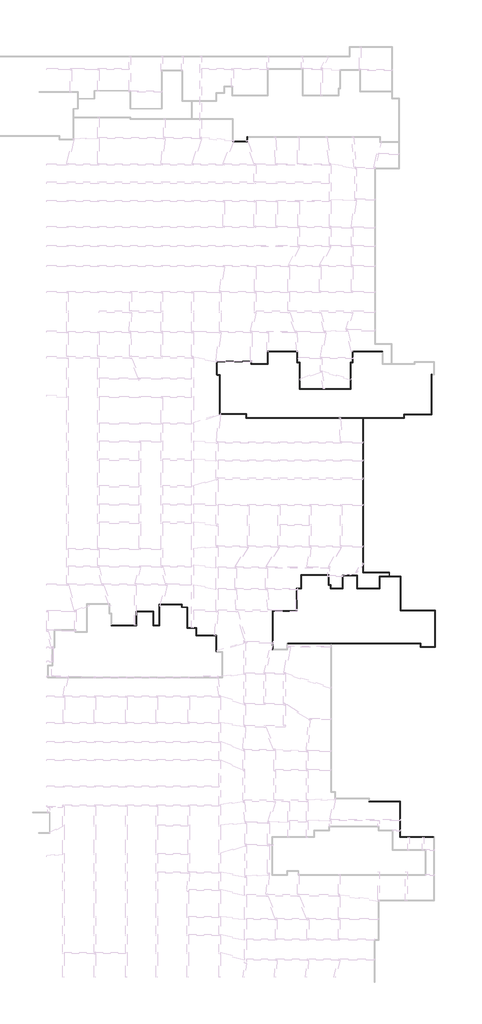
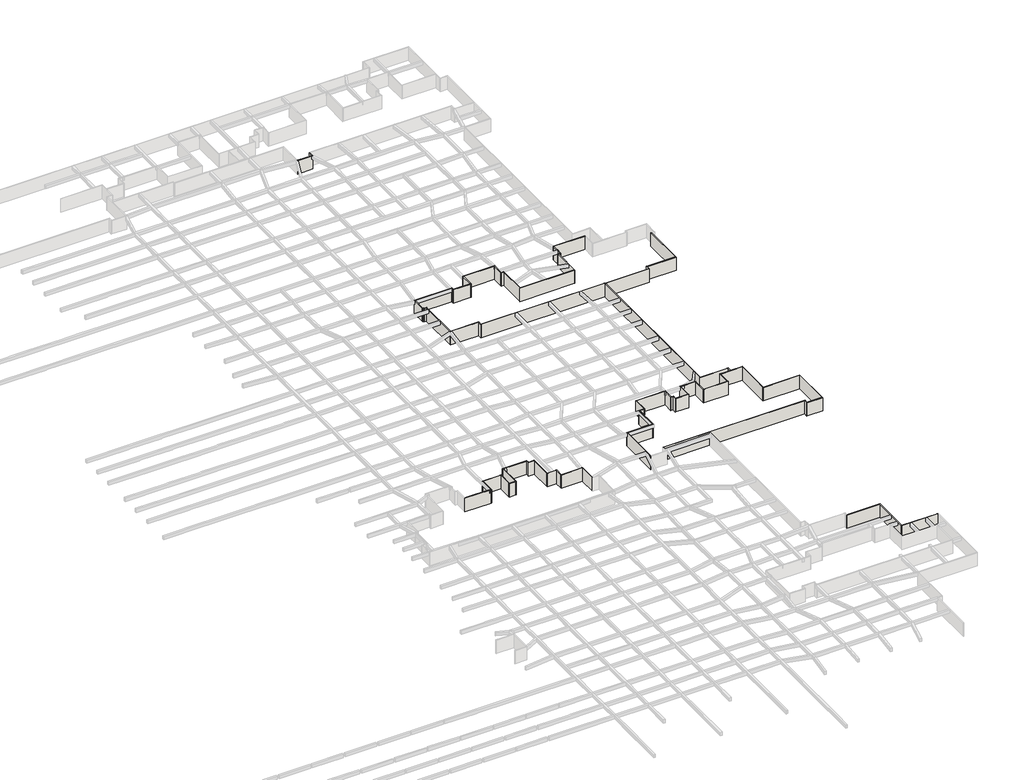
# One storey, part 9 of 45: 69 walls.
"""IFC4 building model written with IfcOpenShell, lengths in millimetres."""

from ifc_helpers import new_model, si_unit, origin, origin_with_axes, place, context, project, spatial, polyline, outline, extrude, faceted_brep, element, save

model = new_model("IFC4")

# Units and contexts
model_context = context("Model", 3, world=origin())
ifc_project = project(units=[si_unit("LENGTHUNIT", "METRE", prefix="MILLI")], contexts=[model_context])

# Site, building, storey
site = spatial("IfcSite", under=ifc_project)
building = spatial("IfcBuilding", under=site)
storey = spatial("IfcBuildingStorey", under=building, Name="户型图", Elevation=0.0)

# Walls
placement = place(None, origin())
element("IfcWall", 1, ObjectType="所有墙体", at=placement, inside=storey, context=model_context, shape_type="Brep", body=[
    faceted_brep([(78199.4783436, 16231.9876735, 0.0), (69819.4783436, 16231.9876735, 0.0), (69699.4783436, 16231.9876735, 0.0), (69699.4783436, 16231.9876735, 3300.0), (69819.4783436, 16231.9876735, 3300.0), (78199.4783436, 16231.9876735, 3300.0), (78199.4783436, 16111.9876735, 0.0), (78199.4783436, 16111.9876735, 3300.0), (69699.4783436, 16111.9876735, 3300.0), (69699.4783436, 16111.9876735, 0.0)], [[[0, 1, 2, 3, 4, 5]], [[6, 7, 8, 9]], [[2, 1, 0, 6, 9]], [[5, 4, 3, 8, 7]], [[0, 5, 7, 6]], [[3, 2, 9, 8]]]),
])
element("IfcWall", 2, ObjectType="所有墙体", at=placement, inside=storey, context=model_context, shape_type="Brep", body=[
    faceted_brep([(69819.4783436, 16231.9876735, 0.0), (69819.4783436, 25131.9876735, 0.0), (69819.4783436, 25131.9876735, 3300.0), (69819.4783436, 16231.9876735, 3300.0), (69699.4783436, 16231.9876735, 0.0), (69699.4783436, 16231.9876735, 3300.0), (69699.4783436, 25011.9876735, 3300.0), (69699.4783436, 25131.9876735, 3300.0), (69699.4783436, 25131.9876735, 0.0), (69699.4783436, 25011.9876735, 0.0)], [[[0, 1, 2, 3]], [[4, 5, 6, 7, 8, 9]], [[1, 0, 4, 9, 8]], [[3, 2, 7, 6, 5]], [[0, 3, 5, 4]], [[2, 1, 8, 7]]]),
])
element("IfcWall", 3, ObjectType="所有墙体", at=placement, inside=storey, context=model_context, shape_type="Brep", body=[
    faceted_brep([(69699.4783436, 25131.9876735, 0.0), (62019.4783436, 25131.9876735, 0.0), (61899.4783436, 25131.9876735, 0.0), (61899.4783436, 25131.9876735, 3300.0), (62019.4783436, 25131.9876735, 3300.0), (69699.4783436, 25131.9876735, 3300.0), (69699.4783436, 25011.9876735, 0.0), (69699.4783436, 25011.9876735, 3300.0), (61899.4783436, 25011.9876735, 3300.0), (61899.4783436, 25011.9876735, 0.0)], [[[0, 1, 2, 3, 4, 5]], [[6, 7, 8, 9]], [[2, 1, 0, 6, 9]], [[5, 4, 3, 8, 7]], [[0, 5, 7, 6]], [[3, 2, 9, 8]]]),
])
element("IfcWall", 4, ObjectType="所有墙体", at=placement, inside=storey, context=model_context, shape_type="Brep", body=[
    faceted_brep([(41607.3862954, 64511.9876735, 0.0), (52399.4783436, 64511.9876735, 0.0), (52519.4783436, 64511.9876735, 0.0), (74799.4783436, 64511.9876735, 0.0), (74919.4783436, 64511.9876735, 0.0), (74919.4783436, 64511.9876735, 3300.0), (74799.4783436, 64511.9876735, 3300.0), (52519.4783436, 64511.9876735, 3300.0), (52399.4783436, 64511.9876735, 3300.0), (41607.3862954, 64511.9876735, 3300.0), (41607.3862954, 64631.9876735, 0.0), (41607.3862954, 64631.9876735, 3300.0), (74919.4783436, 64631.9876735, 3300.0), (74919.4783436, 64631.9876735, 0.0)], [[[0, 1, 2, 3, 4, 5, 6, 7, 8, 9]], [[10, 11, 12, 13]], [[4, 3, 2, 1, 0, 10, 13]], [[9, 8, 7, 6, 5, 12, 11]], [[5, 4, 13, 12]], [[0, 9, 11, 10]]]),
])
element("IfcWall", 5, ObjectType="所有墙体", at=placement, inside=storey, context=model_context, shape_type="Brep", body=[
    faceted_brep([(74799.4783436, 64511.9876735, 0.0), (74799.4783436, 63611.9876735, 0.0), (74799.4783436, 63611.9876735, 3300.0), (74799.4783436, 64511.9876735, 3300.0), (74919.4783436, 64511.9876735, 0.0), (74919.4783436, 64511.9876735, 3300.0), (74919.4783436, 63731.9876735, 3300.0), (74919.4783436, 63611.9876735, 3300.0), (74919.4783436, 63611.9876735, 0.0), (74919.4783436, 63731.9876735, 0.0)], [[[0, 1, 2, 3]], [[4, 5, 6, 7, 8, 9]], [[1, 0, 4, 9, 8]], [[3, 2, 7, 6, 5]], [[0, 3, 5, 4]], [[2, 1, 8, 7]]]),
])
element("IfcWall", 6, ObjectType="所有墙体", at=placement, inside=storey, context=model_context, shape_type="Brep", body=[
    faceted_brep([(74919.4783436, 63611.9876735, 0.0), (78519.4783436, 63611.9876735, 0.0), (78519.4783436, 63611.9876735, 3300.0), (74919.4783436, 63611.9876735, 3300.0), (74919.4783436, 63731.9876735, 0.0), (74919.4783436, 63731.9876735, 3300.0), (78399.4783436, 63731.9876735, 3300.0), (78519.4783436, 63731.9876735, 3300.0), (78519.4783436, 63731.9876735, 0.0), (78399.4783436, 63731.9876735, 0.0)], [[[0, 1, 2, 3]], [[4, 5, 6, 7, 8, 9]], [[1, 0, 4, 9, 8]], [[3, 2, 7, 6, 5]], [[0, 3, 5, 4]], [[2, 1, 8, 7]]]),
])
element("IfcWall", 7, ObjectType="所有墙体", at=placement, inside=storey, context=model_context, shape_type="Brep", body=[
    faceted_brep([(78519.4783436, 63731.9876735, 0.0), (78519.4783436, 72831.9876735, 0.0), (78519.4783436, 72831.9876735, 3300.0), (78519.4783436, 63731.9876735, 3300.0), (78399.4783436, 63731.9876735, 0.0), (78399.4783436, 63731.9876735, 3300.0), (78399.4783436, 72711.9876735, 3300.0), (78399.4783436, 72831.9876735, 3300.0), (78399.4783436, 72831.9876735, 0.0), (78399.4783436, 72711.9876735, 0.0)], [[[0, 1, 2, 3]], [[4, 5, 6, 7, 8, 9]], [[1, 0, 4, 9, 8]], [[3, 2, 7, 6, 5]], [[0, 3, 5, 4]], [[2, 1, 8, 7]]]),
])
element("IfcWall", 8, ObjectType="所有墙体", at=placement, inside=storey, context=model_context, shape_type="Brep", body=[
    faceted_brep([(78399.4783436, 72831.9876735, 0.0), (69919.4783436, 72831.9876735, 0.0), (69799.4783436, 72831.9876735, 0.0), (69799.4783436, 72831.9876735, 3300.0), (69919.4783436, 72831.9876735, 3300.0), (78399.4783436, 72831.9876735, 3300.0), (78399.4783436, 72711.9876735, 0.0), (78399.4783436, 72711.9876735, 3300.0), (69799.4783436, 72711.9876735, 3300.0), (69799.4783436, 72711.9876735, 0.0)], [[[0, 1, 2, 3, 4, 5]], [[6, 7, 8, 9]], [[2, 1, 0, 6, 9]], [[5, 4, 3, 8, 7]], [[0, 5, 7, 6]], [[3, 2, 9, 8]]]),
])
element("IfcWall", 9, ObjectType="所有墙体", at=placement, inside=storey, context=model_context, shape_type="Brep", body=[
    faceted_brep([(69919.4783436, 72831.9876735, 0.0), (69919.4783436, 81331.9876735, 0.0), (69919.4783436, 81331.9876735, 3300.0), (69919.4783436, 72831.9876735, 3300.0), (69799.4783436, 72831.9876735, 0.0), (69799.4783436, 72831.9876735, 3300.0), (69799.4783436, 81211.9876735, 3300.0), (69799.4783436, 81331.9876735, 3300.0), (69799.4783436, 81331.9876735, 0.0), (69799.4783436, 81211.9876735, 0.0)], [[[0, 1, 2, 3]], [[4, 5, 6, 7, 8, 9]], [[1, 0, 4, 9, 8]], [[3, 2, 7, 6, 5]], [[0, 3, 5, 4]], [[2, 1, 8, 7]]]),
])
element("IfcWall", 10, ObjectType="所有墙体", at=placement, inside=storey, context=model_context, shape_type="Brep", body=[
    faceted_brep([(69799.4783436, 81331.9876735, 0.0), (67119.4783436, 81331.9876735, 0.0), (66999.4783436, 81331.9876735, 0.0), (64738.2147368, 81331.9876735, 0.0), (64738.2147368, 81331.9876735, 3300.0), (66999.4783436, 81331.9876735, 3300.0), (67119.4783436, 81331.9876735, 3300.0), (69799.4783436, 81331.9876735, 3300.0), (69799.4783436, 81211.9876735, 0.0), (69799.4783436, 81211.9876735, 3300.0), (64738.2147368, 81211.9876735, 3300.0), (64738.2147368, 81211.9876735, 0.0)], [[[0, 1, 2, 3, 4, 5, 6, 7]], [[8, 9, 10, 11]], [[3, 2, 1, 0, 8, 11]], [[7, 6, 5, 4, 10, 9]], [[0, 7, 9, 8]], [[4, 3, 11, 10]]]),
])
element("IfcWall", 11, ObjectType="所有墙体", at=placement, inside=storey, context=model_context, shape_type="Brep", body=[
    faceted_brep([(67119.4783436, 81331.9876735, 0.0), (67119.4783436, 82331.9876735, 0.0), (67119.4783436, 82331.9876735, 3300.0), (67119.4783436, 81331.9876735, 3300.0), (66999.4783436, 81331.9876735, 0.0), (66999.4783436, 81331.9876735, 3300.0), (66999.4783436, 82211.9876735, 3300.0), (66999.4783436, 82331.9876735, 3300.0), (66999.4783436, 82331.9876735, 0.0), (66999.4783436, 82211.9876735, 0.0)], [[[0, 1, 2, 3]], [[4, 5, 6, 7, 8, 9]], [[1, 0, 4, 9, 8]], [[3, 2, 7, 6, 5]], [[0, 3, 5, 4]], [[2, 1, 8, 7]]]),
])
element("IfcWall", 12, ObjectType="所有墙体", at=placement, inside=storey, context=model_context, shape_type="Brep", body=[
    faceted_brep([(66999.4783436, 82331.9876735, 0.0), (60519.4783436, 82331.9876735, 0.0), (60399.4783436, 82331.9876735, 0.0), (60399.4783436, 82331.9876735, 3300.0), (60519.4783436, 82331.9876735, 3300.0), (66999.4783436, 82331.9876735, 3300.0), (66999.4783436, 82211.9876735, 0.0), (66999.4783436, 82211.9876735, 3300.0), (60399.4783436, 82211.9876735, 3300.0), (60399.4783436, 82211.9876735, 0.0)], [[[0, 1, 2, 3, 4, 5]], [[6, 7, 8, 9]], [[2, 1, 0, 6, 9]], [[5, 4, 3, 8, 7]], [[0, 5, 7, 6]], [[3, 2, 9, 8]]]),
])
element("IfcWall", 13, ObjectType="所有墙体", at=placement, inside=storey, context=model_context, shape_type="Brep", body=[
    faceted_brep([(60519.4783436, 82331.9876735, 0.0), (60519.4783436, 120811.9876735, 0.0), (60519.4783436, 120931.9876735, 0.0), (60519.4783436, 120931.9876735, 3300.0), (60519.4783436, 120811.9876735, 3300.0), (60519.4783436, 82331.9876735, 3300.0), (60399.4783436, 82331.9876735, 0.0), (60399.4783436, 82331.9876735, 3300.0), (60399.4783436, 120846.7035402, 3300.0), (60399.4783436, 120931.9876735, 3300.0), (60399.4783436, 120931.9876735, 0.0), (60399.4783436, 120846.7035402, 0.0)], [[[0, 1, 2, 3, 4, 5]], [[6, 7, 8, 9, 10, 11]], [[2, 1, 0, 6, 11, 10]], [[5, 4, 3, 9, 8, 7]], [[0, 5, 7, 6]], [[3, 2, 10, 9]]]),
])
element("IfcWall", 14, ObjectType="所有墙体", at=placement, inside=storey, context=model_context, shape_type="Brep", body=[
    faceted_brep([(60519.4783436, 120811.9876735, 0.0), (70819.4783436, 120811.9876735, 0.0), (70819.4783436, 120811.9876735, 3300.0), (60519.4783436, 120811.9876735, 3300.0), (60519.4783436, 120931.9876735, 0.0), (60519.4783436, 120931.9876735, 3300.0), (70699.4783436, 120931.9876735, 3300.0), (70819.4783436, 120931.9876735, 3300.0), (70819.4783436, 120931.9876735, 0.0), (70699.4783436, 120931.9876735, 0.0)], [[[0, 1, 2, 3]], [[4, 5, 6, 7, 8, 9]], [[1, 0, 4, 9, 8]], [[3, 2, 7, 6, 5]], [[0, 3, 5, 4]], [[2, 1, 8, 7]]]),
])
element("IfcWall", 15, ObjectType="所有墙体", at=placement, inside=storey, context=model_context, shape_type="Brep", body=[
    faceted_brep([(70819.4783436, 120931.9876735, 0.0), (70819.4783436, 121711.9876735, 0.0), (70819.4783436, 121831.9876735, 0.0), (70819.4783436, 121831.9876735, 3300.0), (70819.4783436, 121711.9876735, 3300.0), (70819.4783436, 120931.9876735, 3300.0), (70699.4783436, 120931.9876735, 0.0), (70699.4783436, 120931.9876735, 3300.0), (70699.4783436, 121831.9876735, 3300.0), (70699.4783436, 121831.9876735, 0.0)], [[[0, 1, 2, 3, 4, 5]], [[6, 7, 8, 9]], [[2, 1, 0, 6, 9]], [[5, 4, 3, 8, 7]], [[0, 5, 7, 6]], [[3, 2, 9, 8]]]),
])
element("IfcWall", 16, ObjectType="所有墙体", at=placement, inside=storey, context=model_context, shape_type="Brep", body=[
    faceted_brep([(70819.4783436, 121711.9876735, 0.0), (77619.4783436, 121711.9876735, 0.0), (77619.4783436, 121711.9876735, 3300.0), (70819.4783436, 121711.9876735, 3300.0), (70819.4783436, 121831.9876735, 0.0), (70819.4783436, 121831.9876735, 3300.0), (77499.4783436, 121831.9876735, 3300.0), (77619.4783436, 121831.9876735, 3300.0), (77619.4783436, 121831.9876735, 0.0), (77499.4783436, 121831.9876735, 0.0)], [[[0, 1, 2, 3]], [[4, 5, 6, 7, 8, 9]], [[1, 0, 4, 9, 8]], [[3, 2, 7, 6, 5]], [[0, 3, 5, 4]], [[2, 1, 8, 7]]]),
])
element("IfcWall", 17, ObjectType="所有墙体", at=placement, inside=storey, context=model_context, shape_type="Brep", body=[
    faceted_brep([(77619.4783436, 121831.9876735, 0.0), (77619.4783436, 131611.9876735, 0.0), (77619.4783436, 131731.9876735, 0.0), (77619.4783436, 131731.9876735, 3300.0), (77619.4783436, 131611.9876735, 3300.0), (77619.4783436, 121831.9876735, 3300.0), (77499.4783436, 121831.9876735, 0.0), (77499.4783436, 121831.9876735, 3300.0), (77499.4783436, 131731.9876735, 3300.0), (77499.4783436, 131731.9876735, 0.0)], [[[0, 1, 2, 3, 4, 5]], [[6, 7, 8, 9]], [[2, 1, 0, 6, 9]], [[5, 4, 3, 8, 7]], [[0, 5, 7, 6]], [[3, 2, 9, 8]]]),
])
element("IfcWall", 18, ObjectType="所有墙体", at=placement, inside=storey, context=model_context, shape_type="Brep", body=[
    faceted_brep([(27971.0399311, 189831.009409, 0.0), (31556.641355, 189831.009409, 0.0), (31556.641355, 189831.009409, 3300.0), (27971.0399311, 189831.009409, 3300.0), (27971.0399311, 189951.009409, 0.0), (27971.0399311, 189951.009409, 3300.0), (31436.641355, 189951.009409, 3300.0), (31556.641355, 189951.009409, 3300.0), (31556.641355, 189951.009409, 0.0), (31436.641355, 189951.009409, 0.0)], [[[0, 1, 2, 3]], [[4, 5, 6, 7, 8, 9]], [[1, 0, 4, 9, 8]], [[3, 2, 7, 6, 5]], [[0, 3, 5, 4]], [[2, 1, 8, 7]]]),
])
element("IfcWall", 19, ObjectType="所有墙体", at=placement, inside=storey, context=model_context, shape_type="Brep", body=[
    faceted_brep([(31556.641355, 189951.009409, 0.0), (31556.641355, 191031.009409, 0.0), (31556.641355, 191151.009409, 0.0), (31556.641355, 191151.009409, 3300.0), (31556.641355, 191031.009409, 3300.0), (31556.641355, 189951.009409, 3300.0), (31436.641355, 189951.009409, 0.0), (31436.641355, 189951.009409, 3300.0), (31436.641355, 191151.009409, 3300.0), (31436.641355, 191151.009409, 0.0)], [[[0, 1, 2, 3, 4, 5]], [[6, 7, 8, 9]], [[2, 1, 0, 6, 9]], [[5, 4, 3, 8, 7]], [[0, 5, 7, 6]], [[3, 2, 9, 8]]]),
])
element("IfcWall", 20, ObjectType="所有墙体", at=placement, inside=storey, context=model_context, shape_type="Brep", body=[
    faceted_brep([(23805.9205959, 135031.9876735, 0.0), (23805.9205959, 131823.6321803, 0.0), (23805.9205959, 131823.6321803, 3300.0), (23805.9205959, 135031.9876735, 3300.0), (23925.9205959, 135031.9876735, 0.0), (23925.9205959, 135031.9876735, 3300.0), (23925.9205959, 134911.9876735, 3300.0), (23925.9205959, 131823.6321803, 3300.0), (23925.9205959, 131823.6321803, 0.0), (23925.9205959, 134911.9876735, 0.0)], [[[0, 1, 2, 3]], [[4, 5, 6, 7, 8, 9]], [[1, 0, 4, 9, 8]], [[3, 2, 7, 6, 5]], [[2, 1, 8, 7]], [[0, 3, 5, 4]]]),
])
element("IfcWall", 21, ObjectType="所有墙体", at=placement, inside=storey, context=model_context, shape_type="Brep", body=[
    faceted_brep([(23805.9205959, 131703.6321803, 0.0), (24005.9205959, 131703.6321803, 0.0), (24125.9205959, 131703.6321803, 0.0), (24125.9205959, 131703.6321803, 3300.0), (24005.9205959, 131703.6321803, 3300.0), (23805.9205959, 131703.6321803, 3300.0), (23805.9205959, 131823.6321803, 0.0), (23805.9205959, 131823.6321803, 3300.0), (23925.9205959, 131823.6321803, 3300.0), (24125.9205959, 131823.6321803, 3300.0), (24125.9205959, 131823.6321803, 0.0), (23925.9205959, 131823.6321803, 0.0)], [[[0, 1, 2, 3, 4, 5]], [[6, 7, 8, 9, 10, 11]], [[2, 1, 0, 6, 11, 10]], [[5, 4, 3, 9, 8, 7]], [[0, 5, 7, 6]], [[3, 2, 10, 9]]]),
])
element("IfcWall", 22, ObjectType="所有墙体", at=placement, inside=storey, context=model_context, shape_type="Brep", body=[
    faceted_brep([(24005.9205959, 131703.6321803, 0.0), (24005.9205959, 131503.6321803, 0.0), (24005.9205959, 131503.6321803, 3300.0), (24005.9205959, 131703.6321803, 3300.0), (24125.9205959, 131703.6321803, 0.0), (24125.9205959, 131703.6321803, 3300.0), (24125.9205959, 131623.6321803, 3300.0), (24125.9205959, 131503.6321803, 3300.0), (24125.9205959, 131503.6321803, 0.0), (24125.9205959, 131623.6321803, 0.0)], [[[0, 1, 2, 3]], [[4, 5, 6, 7, 8, 9]], [[1, 0, 4, 9, 8]], [[3, 2, 7, 6, 5]], [[0, 3, 5, 4]], [[2, 1, 8, 7]]]),
])
element("IfcWall", 23, ObjectType="所有墙体", at=placement, inside=storey, context=model_context, shape_type="Brep", body=[
    faceted_brep([(24125.9205959, 131503.6321803, 0.0), (24605.9205959, 131503.6321803, 0.0), (24725.9205959, 131503.6321803, 0.0), (24725.9205959, 131503.6321803, 3300.0), (24605.9205959, 131503.6321803, 3300.0), (24125.9205959, 131503.6321803, 3300.0), (24125.9205959, 131623.6321803, 0.0), (24125.9205959, 131623.6321803, 3300.0), (24725.9205959, 131623.6321803, 3300.0), (24725.9205959, 131623.6321803, 0.0)], [[[0, 1, 2, 3, 4, 5]], [[6, 7, 8, 9]], [[2, 1, 0, 6, 9]], [[5, 4, 3, 8, 7]], [[0, 5, 7, 6]], [[3, 2, 9, 8]]]),
])
element("IfcWall", 24, ObjectType="所有墙体", at=placement, inside=storey, context=model_context, shape_type="Brep", body=[
    faceted_brep([(24605.9205959, 131503.6321803, 0.0), (24605.9205959, 121746.7035402, 0.0), (24605.9205959, 121746.7035402, 3300.0), (24605.9205959, 131503.6321803, 3300.0), (24725.9205959, 131503.6321803, 0.0), (24725.9205959, 131503.6321803, 3300.0), (24725.9205959, 121866.7035402, 3300.0), (24725.9205959, 121746.7035402, 3300.0), (24725.9205959, 121746.7035402, 0.0), (24725.9205959, 121866.7035402, 0.0)], [[[0, 1, 2, 3]], [[4, 5, 6, 7, 8, 9]], [[1, 0, 4, 9, 8]], [[3, 2, 7, 6, 5]], [[0, 3, 5, 4]], [[2, 1, 8, 7]]]),
])
element("IfcWall", 25, ObjectType="所有墙体", at=placement, inside=storey, context=model_context, shape_type="Brep", body=[
    faceted_brep([(24725.9205959, 121746.7035402, 0.0), (31205.9205959, 121746.7035402, 0.0), (31325.9205959, 121746.7035402, 0.0), (31325.9205959, 121746.7035402, 3300.0), (31205.9205959, 121746.7035402, 3300.0), (24725.9205959, 121746.7035402, 3300.0), (24725.9205959, 121866.7035402, 0.0), (24725.9205959, 121866.7035402, 3300.0), (31325.9205959, 121866.7035402, 3300.0), (31325.9205959, 121866.7035402, 0.0)], [[[0, 1, 2, 3, 4, 5]], [[6, 7, 8, 9]], [[2, 1, 0, 6, 9]], [[5, 4, 3, 8, 7]], [[0, 5, 7, 6]], [[3, 2, 9, 8]]]),
])
element("IfcWall", 26, ObjectType="所有墙体", at=placement, inside=storey, context=model_context, shape_type="Brep", body=[
    faceted_brep([(31205.9205959, 121746.7035402, 0.0), (31205.9205959, 120846.7035402, 0.0), (31205.9205959, 120846.7035402, 3300.0), (31205.9205959, 121746.7035402, 3300.0), (31325.9205959, 121746.7035402, 0.0), (31325.9205959, 121746.7035402, 3300.0), (31325.9205959, 120966.7035402, 3300.0), (31325.9205959, 120846.7035402, 3300.0), (31325.9205959, 120846.7035402, 0.0), (31325.9205959, 120966.7035402, 0.0)], [[[0, 1, 2, 3]], [[4, 5, 6, 7, 8, 9]], [[1, 0, 4, 9, 8]], [[3, 2, 7, 6, 5]], [[0, 3, 5, 4]], [[2, 1, 8, 7]]]),
])
element("IfcWall", 27, ObjectType="所有墙体", at=placement, inside=storey, context=model_context, shape_type="Brep", body=[
    faceted_brep([(31325.9205959, 120846.7035402, 0.0), (60399.4783436, 120846.7035402, 0.0), (60399.4783436, 120846.7035402, 3300.0), (31325.9205959, 120846.7035402, 3300.0), (31325.9205959, 120966.7035402, 0.0), (31325.9205959, 120966.7035402, 3300.0), (60399.4783436, 120966.7035402, 3300.0), (60399.4783436, 120966.7035402, 0.0), (60399.4783436, 120931.9876735, 0.0), (60399.4783436, 120931.9876735, 3300.0)], [[[0, 1, 2, 3]], [[4, 5, 6, 7]], [[1, 0, 4, 7, 8]], [[3, 2, 9, 6, 5]], [[0, 3, 5, 4]], [[2, 1, 8, 7, 6, 9]]]),
])
element("IfcWall", 28, ObjectType="所有墙体", at=placement, inside=storey, context=model_context, shape_type="Brep", body=[
    faceted_brep([(65299.4783436, 137531.9876735, 0.0), (57865.3118233, 137531.9876735, 0.0), (57865.3118233, 137531.9876735, 3300.0), (65299.4783436, 137531.9876735, 3300.0), (65299.4783436, 137411.9876735, 0.0), (65299.4783436, 137411.9876735, 3300.0), (57985.3118233, 137411.9876735, 3300.0), (57865.3118233, 137411.9876735, 3300.0), (57865.3118233, 137411.9876735, 0.0), (57985.3118233, 137411.9876735, 0.0)], [[[0, 1, 2, 3]], [[4, 5, 6, 7, 8, 9]], [[1, 0, 4, 9, 8]], [[3, 2, 7, 6, 5]], [[0, 3, 5, 4]], [[2, 1, 8, 7]]]),
])
element("IfcWall", 29, ObjectType="所有墙体", at=placement, inside=storey, context=model_context, shape_type="Brep", body=[
    faceted_brep([(57865.3118233, 137411.9876735, 0.0), (57865.3118233, 134731.9876735, 0.0), (57865.3118233, 134611.9876735, 0.0), (57865.3118233, 134611.9876735, 3300.0), (57865.3118233, 134731.9876735, 3300.0), (57865.3118233, 137411.9876735, 3300.0), (57985.3118233, 137411.9876735, 0.0), (57985.3118233, 137411.9876735, 3300.0), (57985.3118233, 134611.9876735, 3300.0), (57985.3118233, 134611.9876735, 0.0)], [[[0, 1, 2, 3, 4, 5]], [[6, 7, 8, 9]], [[2, 1, 0, 6, 9]], [[5, 4, 3, 8, 7]], [[0, 5, 7, 6]], [[3, 2, 9, 8]]]),
])
element("IfcWall", 30, ObjectType="所有墙体", at=placement, inside=storey, context=model_context, shape_type="Brep", body=[
    faceted_brep([(57865.3118233, 134731.9876735, 0.0), (57365.3118233, 134731.9876735, 0.0), (57365.3118233, 134731.9876735, 3300.0), (57865.3118233, 134731.9876735, 3300.0), (57865.3118233, 134611.9876735, 0.0), (57865.3118233, 134611.9876735, 3300.0), (57485.3118233, 134611.9876735, 3300.0), (57365.3118233, 134611.9876735, 3300.0), (57365.3118233, 134611.9876735, 0.0), (57485.3118233, 134611.9876735, 0.0)], [[[0, 1, 2, 3]], [[4, 5, 6, 7, 8, 9]], [[1, 0, 4, 9, 8]], [[3, 2, 7, 6, 5]], [[0, 3, 5, 4]], [[2, 1, 8, 7]]]),
])
element("IfcWall", 31, ObjectType="所有墙体", at=placement, inside=storey, context=model_context, shape_type="Brep", body=[
    faceted_brep([(57365.3118233, 134611.9876735, 0.0), (57365.3118233, 128131.9876735, 0.0), (57365.3118233, 128011.9876735, 0.0), (57365.3118233, 128011.9876735, 3300.0), (57365.3118233, 128131.9876735, 3300.0), (57365.3118233, 134611.9876735, 3300.0), (57485.3118233, 134611.9876735, 0.0), (57485.3118233, 134611.9876735, 3300.0), (57485.3118233, 128011.9876735, 3300.0), (57485.3118233, 128011.9876735, 0.0)], [[[0, 1, 2, 3, 4, 5]], [[6, 7, 8, 9]], [[2, 1, 0, 6, 9]], [[5, 4, 3, 8, 7]], [[0, 5, 7, 6]], [[3, 2, 9, 8]]]),
])
element("IfcWall", 32, ObjectType="所有墙体", at=placement, inside=storey, context=model_context, shape_type="Brep", body=[
    faceted_brep([(57365.3118233, 128131.9876735, 0.0), (44685.3118233, 128131.9876735, 0.0), (44565.3118233, 128131.9876735, 0.0), (44565.3118233, 128131.9876735, 3300.0), (44685.3118233, 128131.9876735, 3300.0), (57365.3118233, 128131.9876735, 3300.0), (57365.3118233, 128011.9876735, 0.0), (57365.3118233, 128011.9876735, 3300.0), (44565.3118233, 128011.9876735, 3300.0), (44565.3118233, 128011.9876735, 0.0)], [[[0, 1, 2, 3, 4, 5]], [[6, 7, 8, 9]], [[2, 1, 0, 6, 9]], [[5, 4, 3, 8, 7]], [[0, 5, 7, 6]], [[3, 2, 9, 8]]]),
])
element("IfcWall", 33, ObjectType="所有墙体", at=placement, inside=storey, context=model_context, shape_type="Brep", body=[
    faceted_brep([(44685.3118233, 128131.9876735, 0.0), (44685.3118233, 134731.9876735, 0.0), (44685.3118233, 134731.9876735, 3300.0), (44685.3118233, 128131.9876735, 3300.0), (44565.3118233, 128131.9876735, 0.0), (44565.3118233, 128131.9876735, 3300.0), (44565.3118233, 134611.9876735, 3300.0), (44565.3118233, 134731.9876735, 3300.0), (44565.3118233, 134731.9876735, 0.0), (44565.3118233, 134611.9876735, 0.0)], [[[0, 1, 2, 3]], [[4, 5, 6, 7, 8, 9]], [[1, 0, 4, 9, 8]], [[3, 2, 7, 6, 5]], [[0, 3, 5, 4]], [[2, 1, 8, 7]]]),
])
element("IfcWall", 34, ObjectType="所有墙体", at=placement, inside=storey, context=model_context, shape_type="Brep", body=[
    faceted_brep([(44565.3118233, 134731.9876735, 0.0), (44085.3118233, 134731.9876735, 0.0), (43965.3118233, 134731.9876735, 0.0), (43965.3118233, 134731.9876735, 3300.0), (44085.3118233, 134731.9876735, 3300.0), (44565.3118233, 134731.9876735, 3300.0), (44565.3118233, 134611.9876735, 0.0), (44565.3118233, 134611.9876735, 3300.0), (43965.3118233, 134611.9876735, 3300.0), (43965.3118233, 134611.9876735, 0.0)], [[[0, 1, 2, 3, 4, 5]], [[6, 7, 8, 9]], [[2, 1, 0, 6, 9]], [[5, 4, 3, 8, 7]], [[0, 5, 7, 6]], [[3, 2, 9, 8]]]),
])
element("IfcWall", 35, ObjectType="所有墙体", at=placement, inside=storey, context=model_context, shape_type="Brep", body=[
    faceted_brep([(44085.3118233, 134731.9876735, 0.0), (44085.3118233, 137531.9876735, 0.0), (44085.3118233, 137531.9876735, 3300.0), (44085.3118233, 134731.9876735, 3300.0), (43965.3118233, 134731.9876735, 0.0), (43965.3118233, 134731.9876735, 3300.0), (43965.3118233, 137411.9876735, 3300.0), (43965.3118233, 137531.9876735, 3300.0), (43965.3118233, 137531.9876735, 0.0), (43965.3118233, 137411.9876735, 0.0)], [[[0, 1, 2, 3]], [[4, 5, 6, 7, 8, 9]], [[1, 0, 4, 9, 8]], [[3, 2, 7, 6, 5]], [[0, 3, 5, 4]], [[2, 1, 8, 7]]]),
])
element("IfcWall", 36, ObjectType="所有墙体", at=placement, inside=storey, context=model_context, shape_type="Brep", body=[
    faceted_brep([(43965.3118233, 137531.9876735, 0.0), (36602.5542012, 137531.9876735, 0.0), (36602.5542012, 137531.9876735, 3300.0), (43965.3118233, 137531.9876735, 3300.0), (43965.3118233, 137411.9876735, 0.0), (43965.3118233, 137411.9876735, 3300.0), (36722.5542012, 137411.9876735, 3300.0), (36602.5542012, 137411.9876735, 3300.0), (36602.5542012, 137411.9876735, 0.0), (36722.5542012, 137411.9876735, 0.0)], [[[0, 1, 2, 3]], [[4, 5, 6, 7, 8, 9]], [[1, 0, 4, 9, 8]], [[3, 2, 7, 6, 5]], [[0, 3, 5, 4]], [[2, 1, 8, 7]]]),
])
element("IfcWall", 37, ObjectType="所有墙体", at=placement, inside=storey, context=model_context, shape_type="Brep", body=[
    faceted_brep([(36602.5542012, 137411.9876735, 0.0), (36602.5542012, 134431.9876735, 0.0), (36602.5542012, 134311.9876735, 0.0), (36602.5542012, 134311.9876735, 3300.0), (36602.5542012, 134431.9876735, 3300.0), (36602.5542012, 137411.9876735, 3300.0), (36722.5542012, 137411.9876735, 0.0), (36722.5542012, 137411.9876735, 3300.0), (36722.5542012, 134311.9876735, 3300.0), (36722.5542012, 134311.9876735, 0.0)], [[[0, 1, 2, 3, 4, 5]], [[6, 7, 8, 9]], [[2, 1, 0, 6, 9]], [[5, 4, 3, 8, 7]], [[0, 5, 7, 6]], [[3, 2, 9, 8]]]),
])
element("IfcWall", 38, ObjectType="所有墙体", at=placement, inside=storey, context=model_context, shape_type="Brep", body=[
    faceted_brep([(36602.5542012, 134431.9876735, 0.0), (32622.5542012, 134431.9876735, 0.0), (32502.5542012, 134431.9876735, 0.0), (32502.5542012, 134431.9876735, 3300.0), (32622.5542012, 134431.9876735, 3300.0), (36602.5542012, 134431.9876735, 3300.0), (36602.5542012, 134311.9876735, 0.0), (36602.5542012, 134311.9876735, 3300.0), (32502.5542012, 134311.9876735, 3300.0), (32502.5542012, 134311.9876735, 0.0)], [[[0, 1, 2, 3, 4, 5]], [[6, 7, 8, 9]], [[2, 1, 0, 6, 9]], [[5, 4, 3, 8, 7]], [[0, 5, 7, 6]], [[3, 2, 9, 8]]]),
])
element("IfcWall", 39, ObjectType="所有墙体", at=placement, inside=storey, context=model_context, shape_type="Brep", body=[
    faceted_brep([(32622.5542012, 134431.9876735, 0.0), (32622.5542012, 135031.9876735, 0.0), (32622.5542012, 135031.9876735, 3300.0), (32622.5542012, 134431.9876735, 3300.0), (32502.5542012, 134431.9876735, 0.0), (32502.5542012, 134431.9876735, 3300.0), (32502.5542012, 134911.9876735, 3300.0), (32502.5542012, 135031.9876735, 3300.0), (32502.5542012, 135031.9876735, 0.0), (32502.5542012, 134911.9876735, 0.0)], [[[0, 1, 2, 3]], [[4, 5, 6, 7, 8, 9]], [[1, 0, 4, 9, 8]], [[3, 2, 7, 6, 5]], [[0, 3, 5, 4]], [[2, 1, 8, 7]]]),
])
element("IfcWall", 40, ObjectType="所有墙体", at=placement, inside=storey, context=model_context, shape_type="SweptSolid", body=[
    extrude(outline(polyline([(23925.9205959, 135031.9876735), (32502.5542012, 135031.9876735), (32502.5542012, 134911.9876735), (23925.9205959, 134911.9876735), (23925.9205959, 135031.9876735)])), origin_with_axes(), (0.0, 0.0, 1.0), 3300.0),
])
element("IfcWall", 41, ObjectType="所有墙体", at=placement, inside=storey, context=model_context, shape_type="Brep", body=[
    faceted_brep([(44987.3862954, 81638.4446559, 0.0), (44987.3862954, 78338.4446559, 0.0), (44987.3862954, 78218.4446559, 0.0), (44987.3862954, 78218.4446559, 3300.0), (44987.3862954, 78338.4446559, 3300.0), (44987.3862954, 81638.4446559, 3300.0), (45107.3862954, 81638.4446559, 0.0), (45107.3862954, 81638.4446559, 3300.0), (45107.3862954, 81518.4446559, 3300.0), (45107.3862954, 78218.4446559, 3300.0), (45107.3862954, 78218.4446559, 0.0), (45107.3862954, 81518.4446559, 0.0)], [[[0, 1, 2, 3, 4, 5]], [[6, 7, 8, 9, 10, 11]], [[2, 1, 0, 6, 11, 10]], [[5, 4, 3, 9, 8, 7]], [[3, 2, 10, 9]], [[0, 5, 7, 6]]]),
])
element("IfcWall", 42, ObjectType="所有墙体", at=placement, inside=storey, context=model_context, shape_type="Brep", body=[
    faceted_brep([(44987.3862954, 78338.4446559, 0.0), (43787.3862954, 78338.4446559, 0.0), (43787.3862954, 78338.4446559, 3300.0), (44987.3862954, 78338.4446559, 3300.0), (44987.3862954, 78218.4446559, 0.0), (44987.3862954, 78218.4446559, 3300.0), (43907.3862954, 78218.4446559, 3300.0), (43787.3862954, 78218.4446559, 3300.0), (43787.3862954, 78218.4446559, 0.0), (43907.3862954, 78218.4446559, 0.0)], [[[0, 1, 2, 3]], [[4, 5, 6, 7, 8, 9]], [[1, 0, 4, 9, 8]], [[3, 2, 7, 6, 5]], [[0, 3, 5, 4]], [[2, 1, 8, 7]]]),
])
element("IfcWall", 43, ObjectType="所有墙体", at=placement, inside=storey, context=model_context, shape_type="Brep", body=[
    faceted_brep([(43787.3862954, 78218.4446559, 0.0), (43787.3862954, 72738.4446559, 0.0), (43787.3862954, 72618.4446559, 0.0), (43787.3862954, 72618.4446559, 3300.0), (43787.3862954, 72738.4446559, 3300.0), (43787.3862954, 78218.4446559, 3300.0), (43907.3862954, 78218.4446559, 0.0), (43907.3862954, 78218.4446559, 3300.0), (43907.3862954, 72618.4446559, 3300.0), (43907.3862954, 72618.4446559, 0.0)], [[[0, 1, 2, 3, 4, 5]], [[6, 7, 8, 9]], [[2, 1, 0, 6, 9]], [[5, 4, 3, 8, 7]], [[0, 5, 7, 6]], [[3, 2, 9, 8]]]),
])
element("IfcWall", 44, ObjectType="所有墙体", at=placement, inside=storey, context=model_context, shape_type="Brep", body=[
    faceted_brep([(43787.3862954, 72738.4446559, 0.0), (37787.3862954, 72738.4446559, 0.0), (37787.3862954, 72738.4446559, 3300.0), (43787.3862954, 72738.4446559, 3300.0), (43787.3862954, 72618.4446559, 0.0), (43787.3862954, 72618.4446559, 3300.0), (37907.3862954, 72618.4446559, 3300.0), (37787.3862954, 72618.4446559, 3300.0), (37787.3862954, 72618.4446559, 0.0), (37907.3862954, 72618.4446559, 0.0)], [[[0, 1, 2, 3]], [[4, 5, 6, 7, 8, 9]], [[1, 0, 4, 9, 8]], [[3, 2, 7, 6, 5]], [[0, 3, 5, 4]], [[2, 1, 8, 7]]]),
])
element("IfcWall", 45, ObjectType="所有墙体", at=placement, inside=storey, context=model_context, shape_type="Brep", body=[
    faceted_brep([(37787.3862954, 72618.4446559, 0.0), (37787.3862954, 63018.4446559, 0.0), (37787.3862954, 63018.4446559, 3300.0), (37787.3862954, 72618.4446559, 3300.0), (37907.3862954, 72618.4446559, 0.0), (37907.3862954, 72618.4446559, 3300.0), (37907.3862954, 63138.4446559, 3300.0), (37907.3862954, 63018.4446559, 3300.0), (37907.3862954, 63018.4446559, 0.0), (37907.3862954, 63138.4446559, 0.0)], [[[0, 1, 2, 3]], [[4, 5, 6, 7, 8, 9]], [[1, 0, 4, 9, 8]], [[3, 2, 7, 6, 5]], [[0, 3, 5, 4]], [[2, 1, 8, 7]]]),
])
element("IfcWall", 46, ObjectType="所有墙体", at=placement, inside=storey, context=model_context, shape_type="Brep", body=[
    faceted_brep([(45107.3862954, 81518.4446559, 0.0), (51818.2147368, 81518.4446559, 0.0), (51938.2147368, 81518.4446559, 0.0), (51938.2147368, 81518.4446559, 3300.0), (51818.2147368, 81518.4446559, 3300.0), (45107.3862954, 81518.4446559, 3300.0), (45107.3862954, 81638.4446559, 0.0), (45107.3862954, 81638.4446559, 3300.0), (51938.2147368, 81638.4446559, 3300.0), (51938.2147368, 81638.4446559, 0.0)], [[[0, 1, 2, 3, 4, 5]], [[6, 7, 8, 9]], [[2, 1, 0, 6, 9]], [[5, 4, 3, 8, 7]], [[0, 5, 7, 6]], [[3, 2, 9, 8]]]),
])
element("IfcWall", 47, ObjectType="所有墙体", at=placement, inside=storey, context=model_context, shape_type="Brep", body=[
    faceted_brep([(51818.2147368, 81518.4446559, 0.0), (51818.2147368, 79118.4446559, 0.0), (51818.2147368, 79118.4446559, 3300.0), (51818.2147368, 81518.4446559, 3300.0), (51938.2147368, 81518.4446559, 0.0), (51938.2147368, 81518.4446559, 3300.0), (51938.2147368, 79238.4446559, 3300.0), (51938.2147368, 79118.4446559, 3300.0), (51938.2147368, 79118.4446559, 0.0), (51938.2147368, 79238.4446559, 0.0)], [[[0, 1, 2, 3]], [[4, 5, 6, 7, 8, 9]], [[1, 0, 4, 9, 8]], [[3, 2, 7, 6, 5]], [[0, 3, 5, 4]], [[2, 1, 8, 7]]]),
])
element("IfcWall", 48, ObjectType="所有墙体", at=placement, inside=storey, context=model_context, shape_type="Brep", body=[
    faceted_brep([(51938.2147368, 79118.4446559, 0.0), (52318.2147368, 79118.4446559, 0.0), (52438.2147368, 79118.4446559, 0.0), (52438.2147368, 79118.4446559, 3300.0), (52318.2147368, 79118.4446559, 3300.0), (51938.2147368, 79118.4446559, 3300.0), (51938.2147368, 79238.4446559, 0.0), (51938.2147368, 79238.4446559, 3300.0), (52438.2147368, 79238.4446559, 3300.0), (52438.2147368, 79238.4446559, 0.0)], [[[0, 1, 2, 3, 4, 5]], [[6, 7, 8, 9]], [[2, 1, 0, 6, 9]], [[5, 4, 3, 8, 7]], [[0, 5, 7, 6]], [[3, 2, 9, 8]]]),
])
element("IfcWall", 49, ObjectType="所有墙体", at=placement, inside=storey, context=model_context, shape_type="Brep", body=[
    faceted_brep([(52318.2147368, 79118.4446559, 0.0), (52318.2147368, 78218.4446559, 0.0), (52318.2147368, 78218.4446559, 3300.0), (52318.2147368, 79118.4446559, 3300.0), (52438.2147368, 79118.4446559, 0.0), (52438.2147368, 79118.4446559, 3300.0), (52438.2147368, 78338.4446559, 3300.0), (52438.2147368, 78218.4446559, 3300.0), (52438.2147368, 78218.4446559, 0.0), (52438.2147368, 78338.4446559, 0.0)], [[[0, 1, 2, 3]], [[4, 5, 6, 7, 8, 9]], [[1, 0, 4, 9, 8]], [[3, 2, 7, 6, 5]], [[0, 3, 5, 4]], [[2, 1, 8, 7]]]),
])
element("IfcWall", 50, ObjectType="所有墙体", at=placement, inside=storey, context=model_context, shape_type="Brep", body=[
    faceted_brep([(52438.2147368, 78218.4446559, 0.0), (55438.2147368, 78218.4446559, 0.0), (55438.2147368, 78218.4446559, 3300.0), (52438.2147368, 78218.4446559, 3300.0), (52438.2147368, 78338.4446559, 0.0), (52438.2147368, 78338.4446559, 3300.0), (55318.2147368, 78338.4446559, 3300.0), (55438.2147368, 78338.4446559, 3300.0), (55438.2147368, 78338.4446559, 0.0), (55318.2147368, 78338.4446559, 0.0)], [[[0, 1, 2, 3]], [[4, 5, 6, 7, 8, 9]], [[1, 0, 4, 9, 8]], [[3, 2, 7, 6, 5]], [[0, 3, 5, 4]], [[2, 1, 8, 7]]]),
])
element("IfcWall", 51, ObjectType="所有墙体", at=placement, inside=storey, context=model_context, shape_type="Brep", body=[
    faceted_brep([(55438.2147368, 78338.4446559, 0.0), (55438.2147368, 81418.4446559, 0.0), (55438.2147368, 81538.4446559, 0.0), (55438.2147368, 81538.4446559, 3300.0), (55438.2147368, 81418.4446559, 3300.0), (55438.2147368, 78338.4446559, 3300.0), (55318.2147368, 78338.4446559, 0.0), (55318.2147368, 78338.4446559, 3300.0), (55318.2147368, 81538.4446559, 3300.0), (55318.2147368, 81538.4446559, 0.0)], [[[0, 1, 2, 3, 4, 5]], [[6, 7, 8, 9]], [[2, 1, 0, 6, 9]], [[5, 4, 3, 8, 7]], [[0, 5, 7, 6]], [[3, 2, 9, 8]]]),
])
element("IfcWall", 52, ObjectType="所有墙体", at=placement, inside=storey, context=model_context, shape_type="Brep", body=[
    faceted_brep([(55438.2147368, 81418.4446559, 0.0), (58918.2147368, 81418.4446559, 0.0), (59038.2147368, 81418.4446559, 0.0), (59038.2147368, 81418.4446559, 3300.0), (58918.2147368, 81418.4446559, 3300.0), (55438.2147368, 81418.4446559, 3300.0), (55438.2147368, 81538.4446559, 0.0), (55438.2147368, 81538.4446559, 3300.0), (59038.2147368, 81538.4446559, 3300.0), (59038.2147368, 81538.4446559, 0.0)], [[[0, 1, 2, 3, 4, 5]], [[6, 7, 8, 9]], [[2, 1, 0, 6, 9]], [[5, 4, 3, 8, 7]], [[0, 5, 7, 6]], [[3, 2, 9, 8]]]),
])
element("IfcWall", 53, ObjectType="所有墙体", at=placement, inside=storey, context=model_context, shape_type="Brep", body=[
    faceted_brep([(58918.2147368, 81418.4446559, 0.0), (58918.2147368, 78218.4446559, 0.0), (58918.2147368, 78218.4446559, 3300.0), (58918.2147368, 81418.4446559, 3300.0), (59038.2147368, 81418.4446559, 0.0), (59038.2147368, 81418.4446559, 3300.0), (59038.2147368, 78338.4446559, 3300.0), (59038.2147368, 78218.4446559, 3300.0), (59038.2147368, 78218.4446559, 0.0), (59038.2147368, 78338.4446559, 0.0)], [[[0, 1, 2, 3]], [[4, 5, 6, 7, 8, 9]], [[1, 0, 4, 9, 8]], [[3, 2, 7, 6, 5]], [[0, 3, 5, 4]], [[2, 1, 8, 7]]]),
])
element("IfcWall", 54, ObjectType="所有墙体", at=placement, inside=storey, context=model_context, shape_type="Brep", body=[
    faceted_brep([(59038.2147368, 78218.4446559, 0.0), (64738.2147368, 78218.4446559, 0.0), (64738.2147368, 78218.4446559, 3300.0), (59038.2147368, 78218.4446559, 3300.0), (59038.2147368, 78338.4446559, 0.0), (59038.2147368, 78338.4446559, 3300.0), (64618.2147368, 78338.4446559, 3300.0), (64738.2147368, 78338.4446559, 3300.0), (64738.2147368, 78338.4446559, 0.0), (64618.2147368, 78338.4446559, 0.0)], [[[0, 1, 2, 3]], [[4, 5, 6, 7, 8, 9]], [[1, 0, 4, 9, 8]], [[3, 2, 7, 6, 5]], [[0, 3, 5, 4]], [[2, 1, 8, 7]]]),
])
element("IfcWall", 55, ObjectType="所有墙体", at=placement, inside=storey, context=model_context, shape_type="Brep", body=[
    faceted_brep([(64738.2147368, 78338.4446559, 0.0), (64738.2147368, 81211.9876735, 0.0), (64738.2147368, 81331.9876735, 0.0), (64738.2147368, 81331.9876735, 3300.0), (64738.2147368, 81211.9876735, 3300.0), (64738.2147368, 78338.4446559, 3300.0), (64618.2147368, 78338.4446559, 0.0), (64618.2147368, 78338.4446559, 3300.0), (64618.2147368, 81331.9876735, 3300.0), (64618.2147368, 81331.9876735, 0.0)], [[[0, 1, 2, 3, 4, 5]], [[6, 7, 8, 9]], [[2, 1, 0, 6, 9]], [[5, 4, 3, 8, 7]], [[0, 5, 7, 6]], [[3, 2, 9, 8]]]),
])
element("IfcWall", 56, ObjectType="所有墙体", at=placement, inside=storey, context=model_context, shape_type="Brep", body=[
    faceted_brep([(23787.5629112, 62436.5180379, 0.0), (23787.5629112, 66536.5180379, 0.0), (23787.5629112, 66536.5180379, 3300.0), (23787.5629112, 62436.5180379, 3300.0), (23667.5629112, 62436.5180379, 0.0), (23667.5629112, 62436.5180379, 3300.0), (23667.5629112, 66416.5180379, 3300.0), (23667.5629112, 66536.5180379, 3300.0), (23667.5629112, 66536.5180379, 0.0), (23667.5629112, 66416.5180379, 0.0)], [[[0, 1, 2, 3]], [[4, 5, 6, 7, 8, 9]], [[1, 0, 4, 9, 8]], [[3, 2, 7, 6, 5]], [[0, 3, 5, 4]], [[2, 1, 8, 7]]]),
])
element("IfcWall", 57, ObjectType="所有墙体", at=placement, inside=storey, context=model_context, shape_type="Brep", body=[
    faceted_brep([(23667.5629112, 66536.5180379, 0.0), (18787.5629112, 66536.5180379, 0.0), (18667.5629112, 66536.5180379, 0.0), (18667.5629112, 66536.5180379, 3300.0), (18787.5629112, 66536.5180379, 3300.0), (23667.5629112, 66536.5180379, 3300.0), (23667.5629112, 66416.5180379, 0.0), (23667.5629112, 66416.5180379, 3300.0), (18667.5629112, 66416.5180379, 3300.0), (18667.5629112, 66416.5180379, 0.0)], [[[0, 1, 2, 3, 4, 5]], [[6, 7, 8, 9]], [[2, 1, 0, 6, 9]], [[5, 4, 3, 8, 7]], [[0, 5, 7, 6]], [[3, 2, 9, 8]]]),
])
element("IfcWall", 58, ObjectType="所有墙体", at=placement, inside=storey, context=model_context, shape_type="Brep", body=[
    faceted_brep([(18787.5629112, 66536.5180379, 0.0), (18787.5629112, 68436.5180379, 0.0), (18787.5629112, 68436.5180379, 3300.0), (18787.5629112, 66536.5180379, 3300.0), (18667.5629112, 66536.5180379, 0.0), (18667.5629112, 66536.5180379, 3300.0), (18667.5629112, 68316.5180379, 3300.0), (18667.5629112, 68436.5180379, 3300.0), (18667.5629112, 68436.5180379, 0.0), (18667.5629112, 68316.5180379, 0.0)], [[[0, 1, 2, 3]], [[4, 5, 6, 7, 8, 9]], [[1, 0, 4, 9, 8]], [[3, 2, 7, 6, 5]], [[0, 3, 5, 4]], [[2, 1, 8, 7]]]),
])
element("IfcWall", 59, ObjectType="所有墙体", at=placement, inside=storey, context=model_context, shape_type="Brep", body=[
    faceted_brep([(18667.5629112, 68436.5180379, 0.0), (16587.5629112, 68436.5180379, 0.0), (16467.5629112, 68436.5180379, 0.0), (16467.5629112, 68436.5180379, 3300.0), (16587.5629112, 68436.5180379, 3300.0), (18667.5629112, 68436.5180379, 3300.0), (18667.5629112, 68316.5180379, 0.0), (18667.5629112, 68316.5180379, 3300.0), (16467.5629112, 68316.5180379, 3300.0), (16467.5629112, 68316.5180379, 0.0)], [[[0, 1, 2, 3, 4, 5]], [[6, 7, 8, 9]], [[2, 1, 0, 6, 9]], [[5, 4, 3, 8, 7]], [[0, 5, 7, 6]], [[3, 2, 9, 8]]]),
])
element("IfcWall", 60, ObjectType="所有墙体", at=placement, inside=storey, context=model_context, shape_type="Brep", body=[
    faceted_brep([(16587.5629112, 68436.5180379, 0.0), (16587.5629112, 73636.5180379, 0.0), (16587.5629112, 73636.5180379, 3300.0), (16587.5629112, 68436.5180379, 3300.0), (16467.5629112, 68436.5180379, 0.0), (16467.5629112, 68436.5180379, 3300.0), (16467.5629112, 73516.5180379, 3300.0), (16467.5629112, 73636.5180379, 3300.0), (16467.5629112, 73636.5180379, 0.0), (16467.5629112, 73516.5180379, 0.0)], [[[0, 1, 2, 3]], [[4, 5, 6, 7, 8, 9]], [[1, 0, 4, 9, 8]], [[3, 2, 7, 6, 5]], [[0, 3, 5, 4]], [[2, 1, 8, 7]]]),
])
element("IfcWall", 61, ObjectType="所有墙体", at=placement, inside=storey, context=model_context, shape_type="Brep", body=[
    faceted_brep([(16467.5629112, 73636.5180379, 0.0), (15187.5629112, 73636.5180379, 0.0), (15067.5629112, 73636.5180379, 0.0), (15067.5629112, 73636.5180379, 3300.0), (15187.5629112, 73636.5180379, 3300.0), (16467.5629112, 73636.5180379, 3300.0), (16467.5629112, 73516.5180379, 0.0), (16467.5629112, 73516.5180379, 3300.0), (15067.5629112, 73516.5180379, 3300.0), (15067.5629112, 73516.5180379, 0.0)], [[[0, 1, 2, 3, 4, 5]], [[6, 7, 8, 9]], [[2, 1, 0, 6, 9]], [[5, 4, 3, 8, 7]], [[0, 5, 7, 6]], [[3, 2, 9, 8]]]),
])
element("IfcWall", 62, ObjectType="所有墙体", at=placement, inside=storey, context=model_context, shape_type="Brep", body=[
    faceted_brep([(15187.5629112, 73636.5180379, 0.0), (15187.5629112, 74336.5180379, 0.0), (15187.5629112, 74336.5180379, 3300.0), (15187.5629112, 73636.5180379, 3300.0), (15067.5629112, 73636.5180379, 0.0), (15067.5629112, 73636.5180379, 3300.0), (15067.5629112, 74216.5180379, 3300.0), (15067.5629112, 74336.5180379, 3300.0), (15067.5629112, 74336.5180379, 0.0), (15067.5629112, 74216.5180379, 0.0)], [[[0, 1, 2, 3]], [[4, 5, 6, 7, 8, 9]], [[1, 0, 4, 9, 8]], [[3, 2, 7, 6, 5]], [[0, 3, 5, 4]], [[2, 1, 8, 7]]]),
])
element("IfcWall", 63, ObjectType="所有墙体", at=placement, inside=storey, context=model_context, shape_type="Brep", body=[
    faceted_brep([(15067.5629112, 74336.5180379, 0.0), (9467.5629112, 74336.5180379, 0.0), (9467.5629112, 74336.5180379, 3300.0), (15067.5629112, 74336.5180379, 3300.0), (15067.5629112, 74216.5180379, 0.0), (15067.5629112, 74216.5180379, 3300.0), (9587.5629112, 74216.5180379, 3300.0), (9467.5629112, 74216.5180379, 3300.0), (9467.5629112, 74216.5180379, 0.0), (9587.5629112, 74216.5180379, 0.0)], [[[0, 1, 2, 3]], [[4, 5, 6, 7, 8, 9]], [[1, 0, 4, 9, 8]], [[3, 2, 7, 6, 5]], [[0, 3, 5, 4]], [[2, 1, 8, 7]]]),
])
element("IfcWall", 64, ObjectType="所有墙体", at=placement, inside=storey, context=model_context, shape_type="Brep", body=[
    faceted_brep([(9467.5629112, 74216.5180379, 0.0), (9467.5629112, 69136.5180379, 0.0), (9467.5629112, 69016.5180379, 0.0), (9467.5629112, 69016.5180379, 3300.0), (9467.5629112, 69136.5180379, 3300.0), (9467.5629112, 74216.5180379, 3300.0), (9587.5629112, 74216.5180379, 0.0), (9587.5629112, 74216.5180379, 3300.0), (9587.5629112, 69016.5180379, 3300.0), (9587.5629112, 69016.5180379, 0.0)], [[[0, 1, 2, 3, 4, 5]], [[6, 7, 8, 9]], [[2, 1, 0, 6, 9]], [[5, 4, 3, 8, 7]], [[0, 5, 7, 6]], [[3, 2, 9, 8]]]),
])
element("IfcWall", 65, ObjectType="所有墙体", at=placement, inside=storey, context=model_context, shape_type="Brep", body=[
    faceted_brep([(9467.5629112, 69136.5180379, 0.0), (8087.5629112, 69136.5180379, 0.0), (7967.5629112, 69136.5180379, 0.0), (7967.5629112, 69136.5180379, 3300.0), (8087.5629112, 69136.5180379, 3300.0), (9467.5629112, 69136.5180379, 3300.0), (9467.5629112, 69016.5180379, 0.0), (9467.5629112, 69016.5180379, 3300.0), (7967.5629112, 69016.5180379, 3300.0), (7967.5629112, 69016.5180379, 0.0)], [[[0, 1, 2, 3, 4, 5]], [[6, 7, 8, 9]], [[2, 1, 0, 6, 9]], [[5, 4, 3, 8, 7]], [[0, 5, 7, 6]], [[3, 2, 9, 8]]]),
])
element("IfcWall", 66, ObjectType="所有墙体", at=placement, inside=storey, context=model_context, shape_type="Brep", body=[
    faceted_brep([(8087.5629112, 69136.5180379, 0.0), (8087.5629112, 72536.5180379, 0.0), (8087.5629112, 72536.5180379, 3300.0), (8087.5629112, 69136.5180379, 3300.0), (7967.5629112, 69136.5180379, 0.0), (7967.5629112, 69136.5180379, 3300.0), (7967.5629112, 72416.5180379, 3300.0), (7967.5629112, 72536.5180379, 3300.0), (7967.5629112, 72536.5180379, 0.0), (7967.5629112, 72416.5180379, 0.0)], [[[0, 1, 2, 3]], [[4, 5, 6, 7, 8, 9]], [[1, 0, 4, 9, 8]], [[3, 2, 7, 6, 5]], [[0, 3, 5, 4]], [[2, 1, 8, 7]]]),
])
element("IfcWall", 67, ObjectType="所有墙体", at=placement, inside=storey, context=model_context, shape_type="Brep", body=[
    faceted_brep([(7967.5629112, 72536.5180379, 0.0), (3728.0001812, 72536.5180379, 0.0), (3728.0001812, 72536.5180379, 3300.0), (7967.5629112, 72536.5180379, 3300.0), (7967.5629112, 72416.5180379, 0.0), (7967.5629112, 72416.5180379, 3300.0), (3848.0001812, 72416.5180379, 3300.0), (3728.0001812, 72416.5180379, 3300.0), (3728.0001812, 72416.5180379, 0.0), (3848.0001812, 72416.5180379, 0.0)], [[[0, 1, 2, 3]], [[4, 5, 6, 7, 8, 9]], [[1, 0, 4, 9, 8]], [[3, 2, 7, 6, 5]], [[0, 3, 5, 4]], [[2, 1, 8, 7]]]),
])
element("IfcWall", 68, ObjectType="所有墙体", at=placement, inside=storey, context=model_context, shape_type="Brep", body=[
    faceted_brep([(3728.0001812, 72416.5180379, 0.0), (3728.0001812, 69132.5341829, 0.0), (3728.0001812, 69012.5341829, 0.0), (3728.0001812, 69012.5341829, 3300.0), (3728.0001812, 69132.5341829, 3300.0), (3728.0001812, 72416.5180379, 3300.0), (3848.0001812, 72416.5180379, 0.0), (3848.0001812, 72416.5180379, 3300.0), (3848.0001812, 69012.5341829, 3300.0), (3848.0001812, 69012.5341829, 0.0)], [[[0, 1, 2, 3, 4, 5]], [[6, 7, 8, 9]], [[2, 1, 0, 6, 9]], [[5, 4, 3, 8, 7]], [[0, 5, 7, 6]], [[3, 2, 9, 8]]]),
])
element("IfcWall", 69, ObjectType="所有墙体", at=placement, inside=storey, context=model_context, shape_type="Brep", body=[
    faceted_brep([(3728.0001812, 69132.5341829, 0.0), (-2351.9998188, 69132.5341829, 0.0), (-2471.9998188, 69132.5341829, 0.0), (-2471.9998188, 69132.5341829, 3300.0), (-2351.9998188, 69132.5341829, 3300.0), (3728.0001812, 69132.5341829, 3300.0), (3728.0001812, 69012.5341829, 0.0), (3728.0001812, 69012.5341829, 3300.0), (-2471.9998188, 69012.5341829, 3300.0), (-2471.9998188, 69012.5341829, 0.0)], [[[0, 1, 2, 3, 4, 5]], [[6, 7, 8, 9]], [[2, 1, 0, 6, 9]], [[5, 4, 3, 8, 7]], [[0, 5, 7, 6]], [[3, 2, 9, 8]]]),
])

save(model, "model.ifc")

# Revit data of these elements
# Type "所有墙体"
#   Layers, outside or top first: 120 mm "默认" (function 1)
# Elements 1, 2, 3, 4, 5, 6, 7, 8, 9, 10, 11, 12, 13, 14, 15, 16, 17, 18, 19, 20, 21, 22, 23, 24, 25, 26, 27, 28, 29, 30, 31, 32, 33, 34, 35, 36, 37, 38, 39, 40, 41, 42, 43, 44, 45, 46, 47, 48, 49, 50, 51, 52, 53, 54, 55, 56, 57, 58, 59, 60, 61, 62, 63, 64, 65, 66, 67, 68, 69 (IfcWall, "所有墙体")
#   Top Offset = 0 mm
#   Base Offset = 0 mm
#   wall height = 3300 mm
#   Phase Created = 新构造
#   Base Constraint = 户型图
#   Top Constraint = 层高
#   Materials on its faces: "默认"
# Materials
#   "默认": class "其他", colour RGB 192 192 192, transparency 0, Cost = 0
